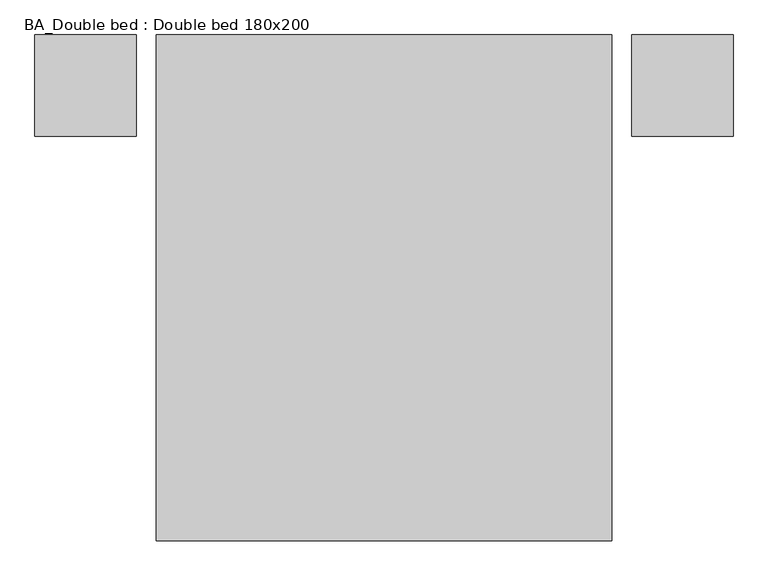
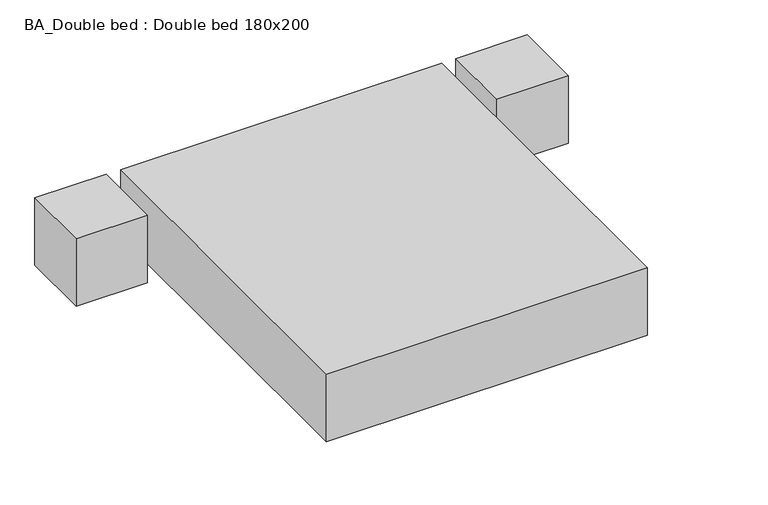
"""IFC4 building model written with IfcOpenShell, lengths in millimetres: furniture geometry, BA_Double bed : Double bed 180x200."""

from ifc_helpers import new_model, si_unit, origin, origin_with_axes, place, context, project, spatial, polyline, outline, extrude, source, transform, mapped, element, save


def ba_double_bed_double_bed_180x200_80237fa8(model_context):
    return source(origin(), model_context, "Body", "SweptSolid", [
        extrude(outline(polyline([(-1380.0, 1000.0), (-980.0, 1000.0), (-980.0, 600.0), (-1380.0, 600.0), (-1380.0, 1000.0)])), origin_with_axes(), (0.0, 0.0, 1.0), 400.0),
        extrude(outline(polyline([(1380.0, 1000.0), (1380.0, 600.0), (980.0, 600.0), (980.0, 1000.0), (1380.0, 1000.0)])), origin_with_axes(), (0.0, 0.0, 1.0), 400.0),
        extrude(outline(polyline([(900.0, 1000.0), (900.0, -1000.0), (-900.0, -1000.0), (-900.0, 1000.0), (900.0, 1000.0)])), origin_with_axes(), (0.0, 0.0, 1.0), 400.0),
    ])


if __name__ == "__main__":
    model = new_model("IFC4")
    model_context = context("Model", 3, world=origin())
    ifc_project = project(units=[si_unit("LENGTHUNIT", "METRE", prefix="MILLI")], contexts=[model_context])
    site = spatial("IfcSite", under=ifc_project)
    building = spatial("IfcBuilding", under=site)
    placement = place(None, origin())
    ba_double_bed_double_bed_180x200_shape = ba_double_bed_double_bed_180x200_80237fa8(model_context)
    element("IfcFurniture", 1, ObjectType="BA_Double bed : Double bed 180x200", at=placement, inside=building, context=model_context, shape_type="MappedRepresentation", body=[
        mapped(ba_double_bed_double_bed_180x200_shape, transform((0.0, 0.0, 0.0), x_axis=(1.0, 0.0, 0.0), y_axis=(0.0, 1.0, 0.0), z_axis=(0.0, 0.0, 1.0))),
    ])
    save(model, "model.ifc")

# Revit data of these elements
# Type "BA_Double bed : Double bed 180x200"
#   width = 1800 mm
#   length = 2000 mm
#   non appearance [instance default] = no
#   appearance [instance default] = yes
#   Default Elevation = 0
# Element 1 (IfcFurniture, "BA_Double bed : Double bed 180x200")
#   Materials on its faces: "Default"
# Materials
#   "Default": class "Generic", colour RGB 255 255 255, transparency 0, Cost = 0
